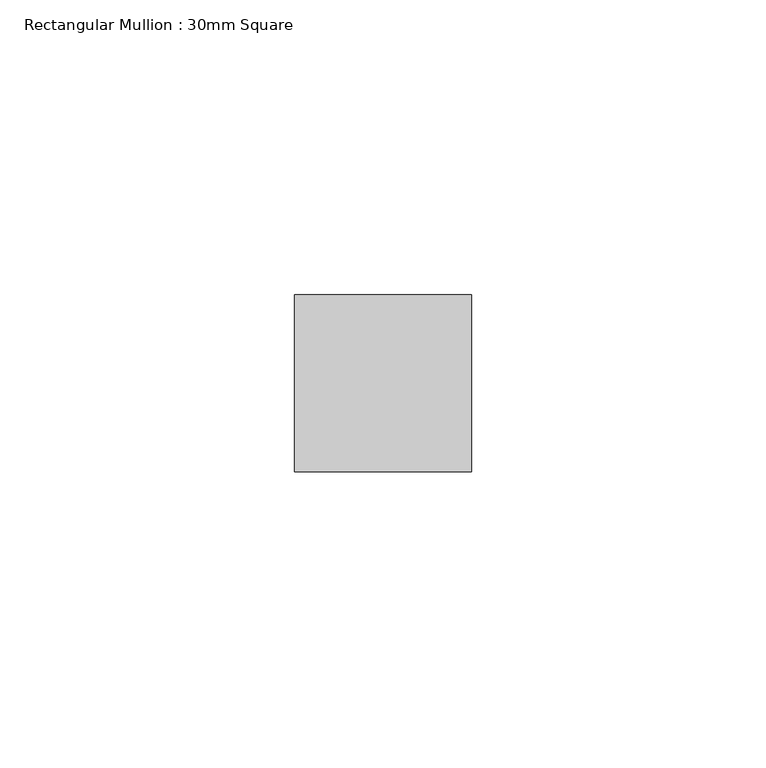
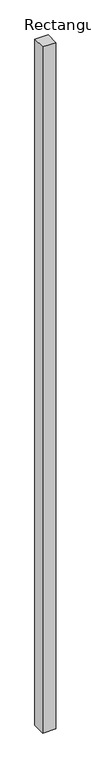
"""IFC4 building model written with IfcOpenShell, lengths in millimetres: member geometry, Rectangular Mullion : 30mm Square."""

from ifc_helpers import new_model, si_unit, frame, origin, place, context, project, spatial, polyline, outline, extrude, source, transform, mapped, element, save


def rectangular_mullion_30mm_square_0a8bdb2b(model_context):
    return source(origin(), model_context, "Body", "SweptSolid", [
        extrude(outline(polyline([(15.0, 15.0), (15.0, -15.0), (-15.0, -15.0), (-15.0, 15.0), (15.0, 15.0)])), frame((0.0, 0.0, -1637.4484709), z_axis=(0.0, 0.0, 1.0), x_axis=(1.0, 0.0, 0.0)), (0.0, 0.0, 1.0), 1637.4484709),
    ])


if __name__ == "__main__":
    model = new_model("IFC4")
    model_context = context("Model", 3, world=origin())
    ifc_project = project(units=[si_unit("LENGTHUNIT", "METRE", prefix="MILLI")], contexts=[model_context])
    site = spatial("IfcSite", under=ifc_project)
    building = spatial("IfcBuilding", under=site)
    placement = place(None, origin())
    rectangular_mullion_30mm_square_shape = rectangular_mullion_30mm_square_0a8bdb2b(model_context)
    element("IfcMember", 1, ObjectType="Rectangular Mullion : 30mm Square", at=placement, inside=building, context=model_context, shape_type="MappedRepresentation", body=[
        mapped(rectangular_mullion_30mm_square_shape, transform((0.0, 0.0, 0.0), x_axis=(1.0, 0.0, 0.0), y_axis=(0.0, 1.0, 0.0), z_axis=(0.0, 0.0, 1.0))),
    ])
    save(model, "model.ifc")

# Revit data of these elements
# Type "Rectangular Mullion : 30mm Square"
#   built-in parameter 1007304 = 0.0984252 (stored number, unit not read)
#   built-in parameter 1007301 = 0.0492126 (stored number, unit not read)
#   built-in parameter 1007300 = 0.0492126 (stored number, unit not read)
# Element 1 (IfcMember, "Rectangular Mullion : 30mm Square")
#   Materials on its faces: "Aluminum"
# Materials
#   "Aluminum": class "Metal", colour RGB 244 244 244, transparency 0, Description = "Aluminum 6061", Cost = 0
